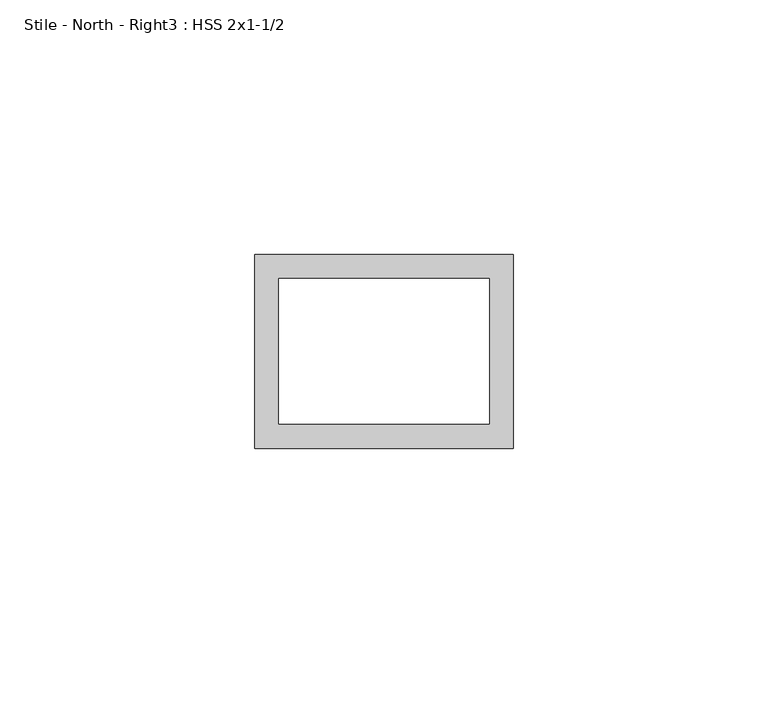
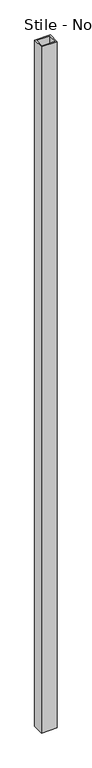
"""IFC4 building model written with IfcOpenShell, lengths in millimetres: proxy geometry, Stile - North - Right3 : HSS 2x1-1/2."""

from ifc_helpers import new_model, si_unit, frame, origin, place, context, project, spatial, polyline, outline, extrude, source, transform, mapped, element, save


def stile_north_right3_hss_2x1_1_2_87095d61(model_context):
    return source(origin(), model_context, "Body", "SweptSolid", [
        extrude(outline(polyline([(587365.8934739, -535163.4663841), (587416.6934739, -535163.4663841), (587416.6934739, -535201.5663841), (587365.8934739, -535201.5663841), (587365.8934739, -535163.4663841)]), holes=[polyline([(587370.6559739, -535168.2288841), (587370.6559739, -535196.8038841), (587411.9309739, -535196.8038841), (587411.9309739, -535168.2288841), (587370.6559739, -535168.2288841)])]), frame((0.0, 0.0, 50.8), z_axis=(0.0, 0.0, 1.0), x_axis=(1.0, 0.0, 0.0)), (0.0, 0.0, 1.0), 2349.5),
    ])


if __name__ == "__main__":
    model = new_model("IFC4")
    model_context = context("Model", 3, world=origin())
    ifc_project = project(units=[si_unit("LENGTHUNIT", "METRE", prefix="MILLI")], contexts=[model_context])
    site = spatial("IfcSite", under=ifc_project)
    building = spatial("IfcBuilding", under=site)
    placement = place(None, origin())
    stile_north_right3_hss_2x1_1_2_shape = stile_north_right3_hss_2x1_1_2_87095d61(model_context)
    element("IfcBuildingElementProxy", 1, Name="Stile - North - Right3 : HSS 2x1-1/2", ObjectType="Stile - North - Right3 : HSS 2x1-1/2", at=placement, inside=building, context=model_context, shape_type="MappedRepresentation", body=[
        mapped(stile_north_right3_hss_2x1_1_2_shape, transform((0.0, 0.0, 0.0), x_axis=(1.0, 0.0, 0.0), y_axis=(0.0, 1.0, 0.0), z_axis=(0.0, 0.0, 1.0))),
    ])
    save(model, "model.ifc")

# Revit data of these elements
# Element 1 (IfcBuildingElementProxy, "Stile - North - Right3 : HSS 2x1-1/2")
#   Materials on its faces: "1-1/2\"X2\" GALV. STL HSS TUBING"
# Materials
#   "1-1/2\"X2\" GALV. STL HSS TUBING": class "Generic", colour RGB 211 211 207, transparency 0, Cost = 0
